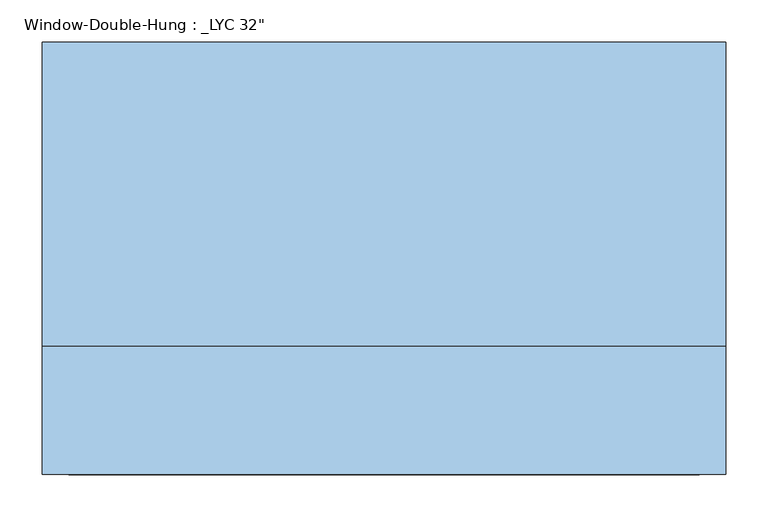
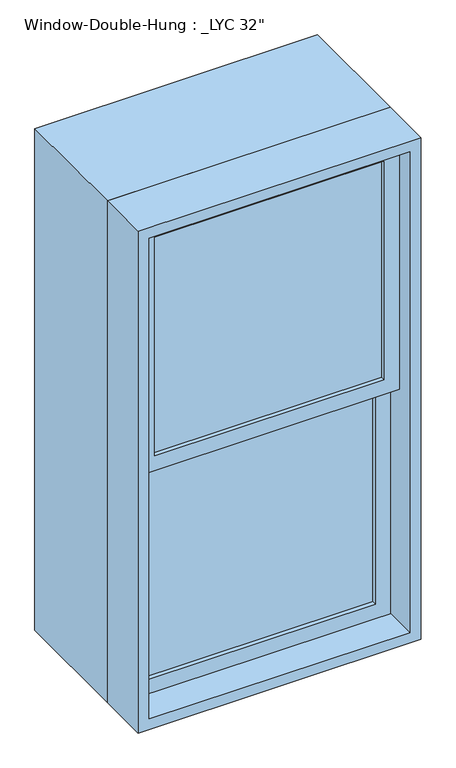
"""IFC4 building model written with IfcOpenShell, lengths in millimetres: window geometry."""

from ifc_helpers import new_model, si_unit, frame, origin, place, context, project, spatial, polyline, outline, extrude, source, transform, mapped, element, save


def window_2b2c187d(model_context):
    return source(origin(), model_context, "Body", "SweptSolid", [
        extrude(outline(polyline([(330.2, -158.75), (-330.2, -158.75), (-330.2, -152.4), (330.2, -152.4), (330.2, -158.75)])), frame((0.0, 0.0, 990.6), z_axis=(0.0, 0.0, 1.0), x_axis=(1.0, 0.0, 0.0)), (0.0, 0.0, 1.0), 663.575),
        extrude(outline(polyline([(-330.2, -146.05), (-330.2, -139.7), (330.2, -139.7), (330.2, -146.05), (-330.2, -146.05)])), frame((0.0, 0.0, 990.6), z_axis=(0.0, 0.0, 1.0), x_axis=(1.0, 0.0, 0.0)), (0.0, 0.0, 1.0), 663.575),
        extrude(outline(polyline([(330.2, -203.2), (-330.2, -203.2), (-330.2, -196.85), (330.2, -196.85), (330.2, -203.2)])), frame((0.0, 0.0, 1698.625), z_axis=(0.0, 0.0, 1.0), x_axis=(1.0, 0.0, 0.0)), (0.0, 0.0, 1.0), 663.575),
        extrude(outline(polyline([(-330.2, -190.5), (-330.2, -184.15), (330.2, -184.15), (330.2, -190.5), (-330.2, -190.5)])), frame((0.0, 0.0, 1698.625), z_axis=(0.0, 0.0, 1.0), x_axis=(1.0, 0.0, 0.0)), (0.0, 0.0, 1.0), 663.575),
        extrude(outline(polyline([(1698.625, 374.65), (1698.625, -374.65), (946.15, -374.65), (946.15, 374.65), (1698.625, 374.65)]), holes=[polyline([(1654.175, -330.2), (1654.175, 330.2), (990.6, 330.2), (990.6, -330.2), (1654.175, -330.2)])]), frame((0.0, -171.45, 0.0), z_axis=(0.0, 1.0, 0.0), x_axis=(0.0, 0.0, 1.0)), (0.0, 0.0, 1.0), 44.45),
        extrude(outline(polyline([(2406.65, 374.65), (2406.65, -374.65), (1654.175, -374.65), (1654.175, 374.65), (2406.65, 374.65)]), holes=[polyline([(2362.2, -330.2), (2362.2, 330.2), (1698.625, 330.2), (1698.625, -330.2), (2362.2, -330.2)])]), frame((0.0, -215.9, 0.0), z_axis=(0.0, 1.0, 0.0), x_axis=(0.0, 0.0, 1.0)), (0.0, 0.0, 1.0), 44.45),
        extrude(outline(polyline([(2438.4, 406.4), (2438.4, -406.4), (914.4, -406.4), (914.4, 406.4), (2438.4, 406.4)]), holes=[polyline([(2406.65, -374.65), (2406.65, 374.65), (946.15, 374.65), (946.15, -374.65), (2406.65, -374.65)])]), frame((0.0, -266.7, 0.0), z_axis=(0.0, 1.0, 0.0), x_axis=(0.0, 0.0, 1.0)), (0.0, 0.0, 1.0), 152.4),
        extrude(outline(polyline([(2438.4, 406.4), (2438.4, -406.4), (914.4, -406.4), (914.4, 406.4), (2438.4, 406.4)]), holes=[polyline([(2419.35, 387.35), (933.45, 387.35), (933.45, -387.35), (2419.35, -387.35), (2419.35, 387.35)])]), frame((0.0, -114.3, 0.0), z_axis=(0.0, 1.0, 0.0), x_axis=(0.0, 0.0, 1.0)), (0.0, 0.0, 1.0), 361.95),
    ])


if __name__ == "__main__":
    model = new_model("IFC4")
    model_context = context("Model", 3, world=origin())
    ifc_project = project(units=[si_unit("LENGTHUNIT", "METRE", prefix="MILLI")], contexts=[model_context])
    site = spatial("IfcSite", under=ifc_project)
    building = spatial("IfcBuilding", under=site)
    placement = place(None, origin())
    window_shape = window_2b2c187d(model_context)
    element("IfcWindow", 1, ObjectType="Window-Double-Hung : _LYC 32\"", at=placement, inside=building, context=model_context, shape_type="MappedRepresentation", body=[
        mapped(window_shape, transform((0.0, 0.0, 0.0), x_axis=(1.0, 0.0, 0.0), y_axis=(0.0, 1.0, 0.0), z_axis=(0.0, 0.0, 1.0))),
    ])
    save(model, "model.ifc")

# Revit data of these elements
# Type "Window-Double-Hung : _LYC 32\""
#   Type Mark = "25"
#   Fire Rating = "0.5h"
#   Assembly Code = "B2020100"
#   Wall Thickness [instance default] = 0' - 6"
#   Visual Light Transmittance = 0.9
#   Thermal Resistance (R) = 1.8146 (h·ft²·°F)/BTU
#   Solar Heat Gain Coefficient = 0.78
#   Rough Width = 2' - 8 1/2"
#   Rough Height = 5' - 0 1/2"
#   Muntin Width = 2' - 2"
#   Muntin Height = 2' - 2 1/8"
#   Interior Wall Closure [instance default] = 0' - 1 1/2"
#   Heat Transfer Coefficient (U) = 0.6496 BTU/(h·ft²·°F)
#   Frame Extension [instance default] = 0' - 2"
#   Exterior Wall Closure [instance default] = 0' - 0 1/2"
#   Extension Jamb [instance default] = 0' - 0 3/4"
#   Height = 5' - 0"
#   Width = 2' - 8"
#   Window Inset [instance default] = 0' - 0 3/4"
#   Top Muntin Visibility = yes
#   Interior Trim Visibility [instance default] = yes
#   Indicator Visibility [instance default] = yes
#   Exterior Trim Visibility [instance default] = yes
#   Extension Jamb Visibility [instance default] = yes
#   Define Thermal Properties by = 1
#   Bottom Muntin Visibility = yes
#   Muntin Pattern = Muntin Pattern_2x2 : Muntin Pattern_2x2
#   Interior Trim Material = Wood - Stained
#   Interior Trim = Trim-Window-Interior-Flat : Picture Frame
#   Interior Frame Material = Wood - Stained
#   Glass Panel Material = Glass
#   Exterior Trim Material = Clad - White
#   Exterior Trim = Trim-Window-Exterior-Flat : with Sill
#   Exterior Frame Material = Clad - White
#   Construction Type Id = ""
#   Wall Closure = (empty or 0)
#   Analytic Construction = (empty or 0)
# Element 1 (IfcWindow, "Window-Double-Hung : _LYC 32\"")
#   Wall Thickness = 1' - 7 1/2"
#   Extension Jamb = 1' - 2 1/4"
#   Materials on its faces: "Wood - Stained", "Glass", "Clad - White"
# Materials
#   "Wood - Stained": class "Wood", colour RGB 224 178 126, transparency 0, Cost = 0
#   "Glass": class "Unassigned", colour RGB 0 128 192, transparency 0.75
#   "Clad - White": class "Wood", colour RGB 242 242 238, transparency 0, Cost = 0
